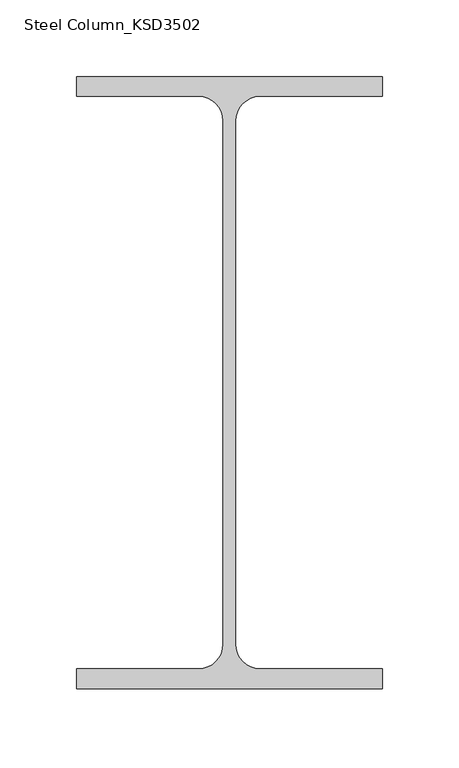
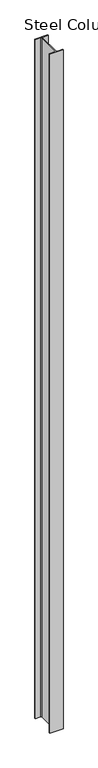
"""IFC4 building model written with IfcOpenShell, lengths in millimetres: column geometry, Steel Column_KSD3502 : H_SC_ASC_H-400×200x8x13."""

from ifc_helpers import new_model, si_unit, point, frame, frame_2d, origin, place, context, project, spatial, polyline, circle_curve, trimmed, segment, composite_curve, outline, extrude, source, transform, mapped, element, save


def steel_column_ksd3502_a45a25b2(model_context):
    return source(origin(), model_context, "Body", "SweptSolid", [
        extrude(outline(composite_curve([segment(polyline([(100.0, 200.0), (100.0, 187.0), (20.0, 187.0)]), True, "CONTINUOUS"), segment(trimmed(circle_curve(frame_2d((20.0, 171.0)), 16.0), [point((20.0, 187.0))], [point((4.0, 171.0))], True, "CARTESIAN"), True, "CONTINUOUS"), segment(polyline([(4.0, 171.0), (4.0, -171.0)]), True, "CONTINUOUS"), segment(trimmed(circle_curve(frame_2d((20.0, -171.0)), 16.0), [point((4.0, -171.0))], [point((20.0, -187.0))], True, "CARTESIAN"), True, "CONTINUOUS"), segment(polyline([(20.0, -187.0), (100.0, -187.0), (100.0, -200.0), (-100.0, -200.0), (-100.0, -187.0), (-20.0, -187.0)]), True, "CONTINUOUS"), segment(trimmed(circle_curve(frame_2d((-20.0, -171.0)), 16.0), [point((-20.0, -187.0))], [point((-4.0, -171.0))], True, "CARTESIAN"), True, "CONTINUOUS"), segment(polyline([(-4.0, -171.0), (-4.0, 171.0)]), True, "CONTINUOUS"), segment(trimmed(circle_curve(frame_2d((-20.0, 171.0)), 16.0), [point((-4.0, 171.0))], [point((-20.0, 187.0))], True, "CARTESIAN"), True, "CONTINUOUS"), segment(polyline([(-20.0, 187.0), (-100.0, 187.0), (-100.0, 200.0), (100.0, 200.0)]), True, "CONTINUOUS")], self_intersect=False)), frame((0.0, 0.0, 6649.9720055), z_axis=(0.0, 0.0, 1.0), x_axis=(1.0, 0.0, 0.0)), (0.0, 0.0, 1.0), 11000.0),
    ])


if __name__ == "__main__":
    model = new_model("IFC4")
    model_context = context("Model", 3, world=origin())
    ifc_project = project(units=[si_unit("LENGTHUNIT", "METRE", prefix="MILLI")], contexts=[model_context])
    site = spatial("IfcSite", under=ifc_project)
    building = spatial("IfcBuilding", under=site)
    placement = place(None, origin())
    steel_column_ksd3502_shape = steel_column_ksd3502_a45a25b2(model_context)
    element("IfcColumn", 1, ObjectType="Steel Column_KSD3502 : H_SC_ASC_H-400×200x8x13", at=placement, inside=building, context=model_context, shape_type="MappedRepresentation", body=[
        mapped(steel_column_ksd3502_shape, transform((0.0, 0.0, 0.0), x_axis=(1.0, 0.0, 0.0), y_axis=(0.0, 1.0, 0.0), z_axis=(0.0, 0.0, 1.0))),
    ])
    save(model, "model.ifc")

# Revit data of these elements
# Type "Steel Column_KSD3502 : H_SC_ASC_H-400×200x8x13"
#   Width = 20.0 cm
#   Web Thickness = 0.8 cm
#   Web Fillet = 1.6 cm
#   Warping Constant = 648999.0 cm⁶
#   Torsional Moment of Inertia = 35.8981 cm⁴
#   Section Area = 84.12 cm²
#   Plastic Modulus weak axis = 268.0 cm³
#   Plastic Modulus strong axis = 1330.0 cm³
#   Perimeter = 1.27 m²/m
#   Nominal Weight = 66.00 kgf/m
#   Moment of Inertia weak axis = 1740.00 cm⁴
#   Moment of Inertia strong axis = 23700.00 cm⁴
#   Height = 40.0 cm
#   Flange Thickness = 1.3 cm
#   Elastic Modulus weak axis = 174.0 cm³
#   Elastic Modulus strong axis = 1190.0 cm³
#   Centroid Vertical = 20.0 cm
#   Centroid Horizontal = 10.0 cm
#   Bolt Spacing = 13.97 cm
#   Structural Material [instance default] = Steel, 45-345
#   Section Name Key = ""
#   Assembly Code = ""
# Element 1 (IfcColumn, "Steel Column_KSD3502 : H_SC_ASC_H-400×200x8x13")
#   Structural Material = none
# Materials
#   "Steel, 45-345": class "Metal", colour RGB 189 187 185, transparency 0, Description = "Steel 345 MPa", Cost = 0
